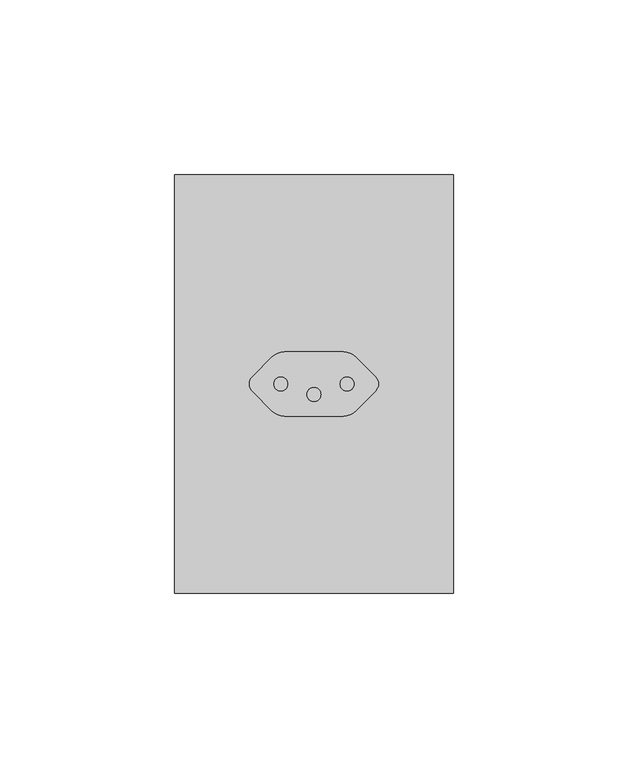
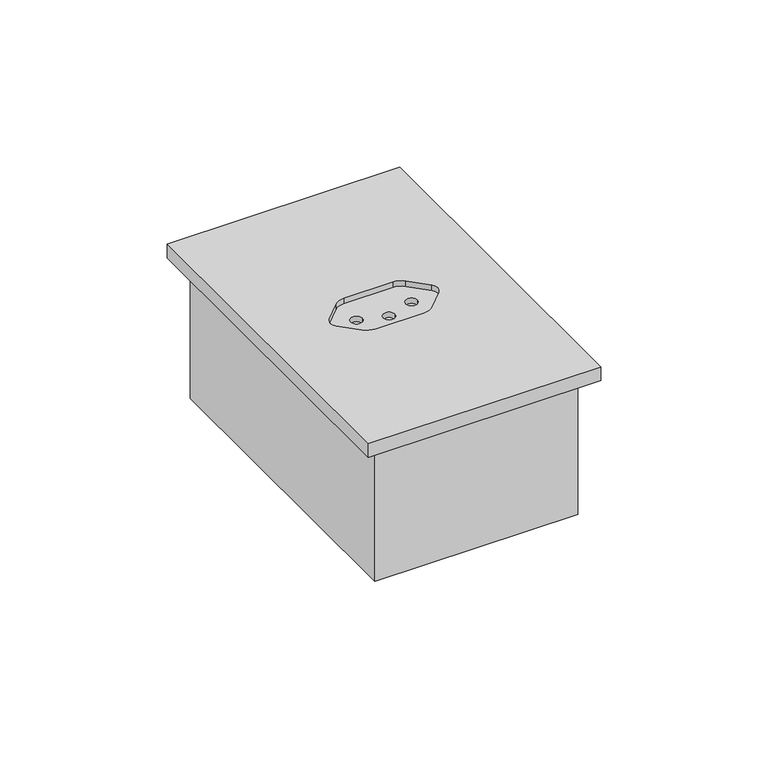
"""IFC4 building model written with IfcOpenShell, lengths in millimetres: proxy geometry, CAIXA VERTICE V7 : Tomada 10A 1s."""

from ifc_helpers import new_model, si_unit, frame, origin, place, context, project, spatial, polyline, circle_curve, faceted_brep, source, transform, mapped, element, save
from ifc_brep_helpers import plane_surface, revolved_surface, advanced_brep


def electrical_fixtures_5046eed1(model_context):
    return source(origin(), model_context, "Body", "SolidModel", [
        faceted_brep([(35.0, -355.0, 0.0), (35.0, -245.0, 0.0), (-35.0, -245.0, 0.0), (-35.0, -355.0, 0.0), (33.0, -353.0, 0.0), (-33.0, -353.0, 0.0), (-33.0, -247.0, 0.0), (33.0, -247.0, 0.0), (33.0, -247.0, -48.0), (-33.0, -247.0, -48.0), (-33.0, -353.0, -48.0), (33.0, -353.0, -48.0), (35.0, -355.0, -50.0), (-35.0, -355.0, -50.0), (-35.0, -245.0, -50.0), (35.0, -245.0, -50.0)], [[[0, 1, 2, 3], [4, 5, 6, 7]], [[8, 9, 10, 11]], [[12, 13, 14, 15]], [[12, 0, 3, 13]], [[3, 2, 14, 13]], [[2, 1, 15, 14]], [[1, 0, 12, 15]], [[7, 8, 11, 4]], [[6, 9, 8, 7]], [[5, 10, 9, 6]], [[4, 11, 10, 5]]]),
        advanced_brep(
        [(40.0, -360.0, 5.0), (40.0, -240.0, 5.0), (-40.0, -240.0, 5.0), (-40.0, -360.0, 5.0), (8.4215729, -290.75, 5.0), (11.9571068, -292.2144661, 5.0), (17.6213203, -297.8786797, 5.0), (17.6213203, -302.1213203, 5.0), (11.9571068, -307.7855339, 5.0), (8.4215729, -309.25, 5.0), (-8.4215729, -309.25, 5.0), (-11.9571068, -307.7855339, 5.0), (-17.6213203, -302.1213203, 5.0), (-17.6213203, -297.8786797, 5.0), (-11.9571068, -292.2144661, 5.0), (-8.4215729, -290.75, 5.0), (-40.0, -360.0, 0.0), (-40.0, -240.0, 0.0), (40.0, -240.0, 0.0), (40.0, -360.0, 0.0), (8.4215729, -290.75, 3.0), (-8.4215729, -290.75, 3.0), (-11.9571068, -292.2144661, 3.0), (-17.6213203, -297.8786797, 3.0), (-17.6213203, -302.1213203, 3.0), (-11.9571068, -307.7855339, 3.0), (-8.4215729, -309.25, 3.0), (8.4215729, -309.25, 3.0), (11.9571068, -307.7855339, 3.0), (17.6213203, -302.1213203, 3.0), (17.6213203, -297.8786797, 3.0), (11.9571068, -292.2144661, 3.0), (-7.5, -300.0, 3.0), (-11.5, -300.0, 3.0), (11.5, -300.0, 3.0), (7.5, -300.0, 3.0), (2.0, -303.0, 3.0), (-2.0, -303.0, 3.0), (-11.5, -300.0, 1.0), (-7.5, -300.0, 1.0), (7.5, -300.0, 1.0), (11.5, -300.0, 1.0), (-2.0, -303.0, 1.0), (2.0, -303.0, 1.0)],
        [
            (0, 1),
            (1, 2),
            (2, 3),
            (3, 0),
            (4, 5, circle_curve(frame((8.4215729, -295.75, 5.0), z_axis=(0.0, 0.0, -1.0), x_axis=(-1.0, 0.0, 0.0)), 5.0)),
            (5, 6),
            (6, 7, circle_curve(frame((15.5, -300.0, 5.0), z_axis=(0.0, 0.0, -1.0), x_axis=(-1.0, 0.0, 0.0)), 3.0)),
            (7, 8),
            (8, 9, circle_curve(frame((8.4215729, -304.25, 5.0), z_axis=(0.0, 0.0, -1.0), x_axis=(-1.0, 0.0, 0.0)), 5.0)),
            (9, 10),
            (10, 11, circle_curve(frame((-8.4215729, -304.25, 5.0), z_axis=(0.0, 0.0, -1.0), x_axis=(-1.0, 0.0, 0.0)), 5.0)),
            (11, 12),
            (12, 13, circle_curve(frame((-15.5, -300.0, 5.0), z_axis=(0.0, 0.0, -1.0), x_axis=(-1.0, 0.0, 0.0)), 3.0)),
            (13, 14),
            (14, 15, circle_curve(frame((-8.4215729, -295.75, 5.0), z_axis=(0.0, 0.0, -1.0), x_axis=(-1.0, 0.0, 0.0)), 5.0)),
            (15, 4),
            (16, 17),
            (17, 18),
            (18, 19),
            (19, 16),
            (3, 16),
            (19, 0),
            (2, 17),
            (1, 18),
            (20, 21),
            (21, 22, circle_curve(frame((-8.4215729, -295.75, 3.0), z_axis=(0.0, 0.0, 1.0), x_axis=(-1.0, 0.0, 0.0)), 5.0)),
            (22, 23),
            (23, 24, circle_curve(frame((-15.5, -300.0, 3.0), z_axis=(0.0, 0.0, 1.0), x_axis=(-1.0, 0.0, 0.0)), 3.0)),
            (24, 25),
            (25, 26, circle_curve(frame((-8.4215729, -304.25, 3.0), z_axis=(0.0, 0.0, 1.0), x_axis=(-1.0, 0.0, 0.0)), 5.0)),
            (26, 27),
            (27, 28, circle_curve(frame((8.4215729, -304.25, 3.0), z_axis=(0.0, 0.0, 1.0), x_axis=(-1.0, 0.0, 0.0)), 5.0)),
            (28, 29),
            (29, 30, circle_curve(frame((15.5, -300.0, 3.0), z_axis=(0.0, 0.0, 1.0), x_axis=(-1.0, 0.0, 0.0)), 3.0)),
            (30, 31),
            (31, 20, circle_curve(frame((8.4215729, -295.75, 3.0), z_axis=(0.0, 0.0, 1.0), x_axis=(-1.0, 0.0, 0.0)), 5.0)),
            (32, 33, circle_curve(frame((-9.5, -300.0, 3.0), z_axis=(0.0, 0.0, -1.0), x_axis=(1.0, -2.301812013077709e-12, 0.0)), 2.0)),
            (33, 32, circle_curve(frame((-9.5, -300.0, 3.0), z_axis=(0.0, 0.0, -1.0), x_axis=(1.0, -2.301812013077709e-12, 0.0)), 2.0)),
            (34, 35, circle_curve(frame((9.5, -300.0, 3.0), z_axis=(0.0, 0.0, -1.0), x_axis=(1.0, -2.301812013077709e-12, 0.0)), 2.0)),
            (35, 34, circle_curve(frame((9.5, -300.0, 3.0), z_axis=(0.0, 0.0, -1.0), x_axis=(1.0, -2.301812013077709e-12, 0.0)), 2.0)),
            (36, 37, circle_curve(frame((0.0, -303.0, 3.0), z_axis=(0.0, 0.0, -1.0), x_axis=(1.0, -2.301812013077709e-12, 0.0)), 2.0)),
            (37, 36, circle_curve(frame((0.0, -303.0, 3.0), z_axis=(0.0, 0.0, -1.0), x_axis=(1.0, -2.301812013077709e-12, 0.0)), 2.0)),
            (20, 4),
            (15, 21),
            (14, 22),
            (13, 23),
            (12, 24),
            (11, 25),
            (10, 26),
            (9, 27),
            (8, 28),
            (7, 29),
            (6, 30),
            (5, 31),
            (38, 39, circle_curve(frame((-9.5, -300.0, 1.0), z_axis=(0.0, 0.0, 1.0), x_axis=(1.0, -2.301812013077709e-12, 0.0)), 2.0)),
            (39, 38, circle_curve(frame((-9.5, -300.0, 1.0), z_axis=(0.0, 0.0, 1.0), x_axis=(1.0, -2.301812013077709e-12, 0.0)), 2.0)),
            (40, 41, circle_curve(frame((9.5, -300.0, 1.0), z_axis=(0.0, 0.0, 1.0), x_axis=(1.0, -2.301812013077709e-12, 0.0)), 2.0)),
            (41, 40, circle_curve(frame((9.5, -300.0, 1.0), z_axis=(0.0, 0.0, 1.0), x_axis=(1.0, -2.301812013077709e-12, 0.0)), 2.0)),
            (42, 43, circle_curve(frame((0.0, -303.0, 1.0), z_axis=(0.0, 0.0, 1.0), x_axis=(1.0, -2.301812013077709e-12, 0.0)), 2.0)),
            (43, 42, circle_curve(frame((0.0, -303.0, 1.0), z_axis=(0.0, 0.0, 1.0), x_axis=(1.0, -2.301812013077709e-12, 0.0)), 2.0)),
            (33, 38),
            (39, 32),
            (35, 40),
            (41, 34),
            (37, 42),
            (43, 36),
        ],
        [
            plane_surface(frame((-60.0, -360.0, 5.0), z_axis=(0.0, 0.0, 1.0), x_axis=(-1.0, 0.0, 0.0))),
            plane_surface(frame((-60.0, -360.0, 0.0), z_axis=(0.0, 0.0, -1.0), x_axis=(1.0, 0.0, 0.0))),
            plane_surface(frame((40.0, -360.0, 5.0), z_axis=(0.0, -1.0, 0.0), x_axis=(0.0, 0.0, -1.0))),
            plane_surface(frame((-40.0, -360.0, 5.0), z_axis=(-1.0, 0.0, 0.0), x_axis=(0.0, 0.0, -1.0))),
            plane_surface(frame((-40.0, -240.0, 5.0), z_axis=(0.0, 1.0, 0.0), x_axis=(0.0, 0.0, -1.0))),
            plane_surface(frame((40.0, -240.0, 5.0), z_axis=(1.0, 0.0, 0.0), x_axis=(0.0, 0.0, -1.0))),
            plane_surface(frame((3.4215729, -295.75, 3.0), z_axis=(0.0, 0.0, 1.0), x_axis=(0.0, -1.0, 0.0))),
            plane_surface(frame((-8.4215729, -290.75, 5.0), z_axis=(0.0, -1.0, 0.0), x_axis=(0.0, 0.0, -1.0))),
            revolved_surface(polyline([(-13.4215729, -295.75, 5.0), (-13.4215729, -295.75, 3.0)]), (-8.4215729, -295.75, 3.0), (0.0, 0.0, 1.0)),
            plane_surface(frame((-17.6213203, -297.8786797, 5.0), z_axis=(0.7071067811865045, -0.7071067811865905, 0.0), x_axis=(0.0, 0.0, -1.0))),
            revolved_surface(polyline([(-18.5, -300.0, 5.0), (-18.5, -300.0, 3.0)]), (-15.5, -300.0, 3.0), (0.0, 0.0, 1.0)),
            plane_surface(frame((-11.9571068, -307.7855339, 5.0), z_axis=(0.7071067811865515, 0.7071067811865437, 0.0), x_axis=(0.0, 0.0, -1.0))),
            revolved_surface(polyline([(-13.4215729, -304.25, 5.0), (-13.4215729, -304.25, 3.0)]), (-8.4215729, -304.25, 3.0), (0.0, 0.0, 1.0)),
            plane_surface(frame((8.4215729, -309.25, 5.0), z_axis=(0.0, 1.0, 0.0), x_axis=(0.0, 0.0, -1.0))),
            revolved_surface(polyline([(3.4215728999999993, -304.25, 5.0), (3.4215728999999993, -304.25, 3.0)]), (8.4215729, -304.25, 3.0), (0.0, 0.0, 1.0)),
            plane_surface(frame((17.6213203, -302.1213203, 5.0), z_axis=(-0.7071067811865307, 0.7071067811865643, 0.0), x_axis=(0.0, 0.0, -1.0))),
            revolved_surface(polyline([(12.5, -300.0, 5.0), (12.5, -300.0, 3.0)]), (15.5, -300.0, 3.0), (0.0, 0.0, 1.0)),
            plane_surface(frame((11.9571068, -292.2144661, 5.0), z_axis=(-0.7071067811865893, -0.7071067811865058, 0.0), x_axis=(0.0, 0.0, -1.0))),
            revolved_surface(polyline([(3.4215728999999993, -295.75, 5.0), (3.4215728999999993, -295.75, 3.0)]), (8.4215729, -295.75, 3.0), (0.0, 0.0, 1.0)),
            plane_surface(frame((-7.5, -300.0, 1.0), z_axis=(0.0, 0.0, 1.0), x_axis=(2.301812013077709e-12, 1.0, 0.0))),
            revolved_surface(polyline([(-7.5, -300.0000000000046, 3.0), (-7.5, -300.0000000000046, 1.0)]), (-9.5, -300.0, 1.0), (0.0, 0.0, 1.0)),
            revolved_surface(polyline([(11.5, -300.0000000000046, 3.0), (11.5, -300.0000000000046, 1.0)]), (9.5, -300.0, 5.0), (0.0, 0.0, 1.0)),
            revolved_surface(polyline([(2.0, -303.0000000000046, 3.0), (2.0, -303.0000000000046, 1.0)]), (0.0, -303.0, 5.0), (0.0, 0.0, 1.0)),
        ],
        [
            (0, [[1, 2, 3, 4], [5, 6, 7, 8, 9, 10, 11, 12, 13, 14, 15, 16]]),
            (1, [[17, 18, 19, 20]]),
            (2, [[21, -20, 22, -4]]),
            (3, [[23, -17, -21, -3]]),
            (4, [[24, -18, -23, -2]]),
            (5, [[-22, -19, -24, -1]]),
            (6, [[25, 26, 27, 28, 29, 30, 31, 32, 33, 34, 35, 36], [37, 38], [39, 40], [41, 42]]),
            (7, [[43, -16, 44, -25]]),
            (8, [[-44, -15, 45, -26]]),
            (9, [[-45, -14, 46, -27]]),
            (10, [[-46, -13, 47, -28]]),
            (11, [[-47, -12, 48, -29]]),
            (12, [[-48, -11, 49, -30]]),
            (13, [[-49, -10, 50, -31]]),
            (14, [[-50, -9, 51, -32]]),
            (15, [[-51, -8, 52, -33]]),
            (16, [[-52, -7, 53, -34]]),
            (17, [[-53, -6, 54, -35]]),
            (18, [[-54, -5, -43, -36]]),
            (19, [[55, 56]]),
            (19, [[57, 58]]),
            (19, [[59, 60]]),
            (20, [[61, -56, 62, -38]]),
            (20, [[-62, -55, -61, -37]]),
            (21, [[63, -58, 64, -40]]),
            (21, [[-64, -57, -63, -39]]),
            (22, [[65, -60, 66, -42]]),
            (22, [[-66, -59, -65, -41]]),
        ],
    ),
    ])


if __name__ == "__main__":
    model = new_model("IFC4")
    model_context = context("Model", 3, world=origin())
    ifc_project = project(units=[si_unit("LENGTHUNIT", "METRE", prefix="MILLI")], contexts=[model_context])
    site = spatial("IfcSite", under=ifc_project)
    building = spatial("IfcBuilding", under=site)
    placement = place(None, origin())
    electrical_fixtures_shape = electrical_fixtures_5046eed1(model_context)
    element("IfcBuildingElementProxy", 1, Name="CAIXA VERTICE V7 : Tomada 10A 1s", ObjectType="CAIXA VERTICE V7 : Tomada 10A 1s", at=placement, inside=building, context=model_context, shape_type="MappedRepresentation", body=[
        mapped(electrical_fixtures_shape, transform((0.0, 0.0, 0.0), x_axis=(1.0, 0.0, 0.0), y_axis=(0.0, 1.0, 0.0), z_axis=(0.0, 0.0, 1.0))),
    ])
    save(model, "model.ifc")

# Revit data of these elements
# Type "CAIXA VERTICE V7 : Tomada 10A 1s"
#   URL = "www.facebook.com/verticetreinamentos"
#   SEÇÃO [instance default] = ""
#   Rotação [instance default] = 0.00°
#   LARGURA DA TAMPA = 0.08 m
#   BORDA = 0.01 m
#   ALTURA DE INSTALAÇÃO [instance default] = 1.10 m
#   Distância Anotação [instance default] = 0.0015 m
#   ALTURA DA TAMPA = 0.12 m
#   Vertical [instance default] = yes
#   VER SEÇÃO [instance default] = no
#   SHADE ESQ [instance default] = no
#   SHADE DIR [instance default] = yes
#   HORIZONTAL [instance default] = no
#   ANDAR COM A LEGENDA [instance default] = 0
#   Material Tampa [instance default] = Plástico, branco opaco
#   Caixa = element 1798514
#   Anotação = element 1798528
#   Default Elevation = 0
# Element 1 (IfcBuildingElementProxy, "CAIXA VERTICE V7 : Tomada 10A 1s")
#   ALTURA DE INSTALAÇÃO = 0.30 m
#   SHADE DIR = no
#   Materials on its faces: "Plástico, branco opaco"
# Materials
#   "Plástico, branco opaco": class "Plástico", colour RGB 120 120 120, transparency 0, Description = "Plastic, generic, opaque white", Cost = 0
